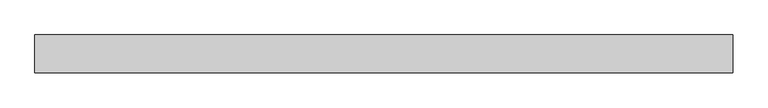
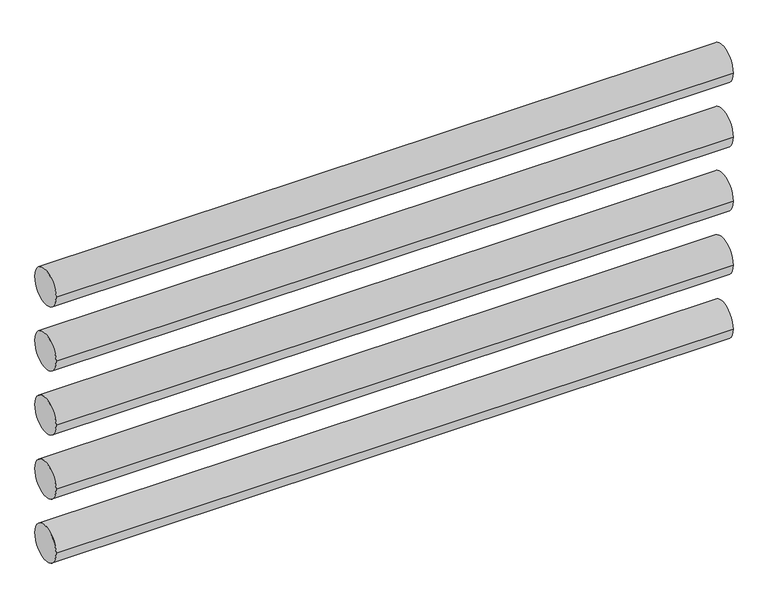
"""IFC4 building model written with IfcOpenShell, lengths in millimetres: proxy geometry, Газпремиум_Регистр : РГТ-2-108х3-2м-5."""

from ifc_helpers import new_model, si_unit, point, frame, frame_2d, origin, place, context, project, spatial, circle_curve, trimmed, segment, composite_curve, outline, extrude, source, transform, mapped, element, save


def mechanical_equipment_43ffbe55(model_context):
    return source(origin(), model_context, "Body", "SweptSolid", [
        extrude(outline(composite_curve([segment(trimmed(circle_curve(frame_2d((0.0, 854.0)), 54.0), [point((-54.0, 854.0))], [point((54.0, 854.0))], False, "CARTESIAN"), True, "CONTINUOUS"), segment(trimmed(circle_curve(frame_2d((0.0, 854.0)), 54.0), [point((54.0, 854.0))], [point((-54.0, 854.0))], False, "CARTESIAN"), True, "CONTINUOUS")], self_intersect=False)), frame((-184.1719207, 0.0, 0.0), z_axis=(1.0, 0.0, 0.0), x_axis=(0.0, 1.0, 0.0)), (0.0, 0.0, 1.0), 2000.0),
        extrude(outline(composite_curve([segment(trimmed(circle_curve(frame_2d((0.0, 654.0)), 54.0), [point((-54.0, 654.0))], [point((54.0, 654.0))], False, "CARTESIAN"), True, "CONTINUOUS"), segment(trimmed(circle_curve(frame_2d((0.0, 654.0)), 54.0), [point((54.0, 654.0))], [point((-54.0, 654.0))], False, "CARTESIAN"), True, "CONTINUOUS")], self_intersect=False)), frame((-184.1719207, 0.0, 0.0), z_axis=(1.0, 0.0, 0.0), x_axis=(0.0, 1.0, 0.0)), (0.0, 0.0, 1.0), 2000.0),
        extrude(outline(composite_curve([segment(trimmed(circle_curve(frame_2d((0.0, 454.0)), 54.0), [point((-54.0, 454.0))], [point((54.0, 454.0))], False, "CARTESIAN"), True, "CONTINUOUS"), segment(trimmed(circle_curve(frame_2d((0.0, 454.0)), 54.0), [point((54.0, 454.0))], [point((-54.0, 454.0))], False, "CARTESIAN"), True, "CONTINUOUS")], self_intersect=False)), frame((-184.1719207, 0.0, 0.0), z_axis=(1.0, 0.0, 0.0), x_axis=(0.0, 1.0, 0.0)), (0.0, 0.0, 1.0), 2000.0),
        extrude(outline(composite_curve([segment(trimmed(circle_curve(frame_2d((0.0, 254.0)), 54.0), [point((-54.0, 254.0))], [point((54.0, 254.0))], False, "CARTESIAN"), True, "CONTINUOUS"), segment(trimmed(circle_curve(frame_2d((0.0, 254.0)), 54.0), [point((54.0, 254.0))], [point((-54.0, 254.0))], False, "CARTESIAN"), True, "CONTINUOUS")], self_intersect=False)), frame((-184.1719207, 0.0, 0.0), z_axis=(1.0, 0.0, 0.0), x_axis=(0.0, 1.0, 0.0)), (0.0, 0.0, 1.0), 2000.0),
        extrude(outline(composite_curve([segment(trimmed(circle_curve(frame_2d((0.0, 54.0)), 54.0), [point((-54.0, 54.0))], [point((54.0, 54.0))], False, "CARTESIAN"), True, "CONTINUOUS"), segment(trimmed(circle_curve(frame_2d((0.0, 54.0)), 54.0), [point((54.0, 54.0))], [point((-54.0, 54.0))], False, "CARTESIAN"), True, "CONTINUOUS")], self_intersect=False)), frame((-184.1719207, 0.0, 0.0), z_axis=(1.0, 0.0, 0.0), x_axis=(0.0, 1.0, 0.0)), (0.0, 0.0, 1.0), 2000.0),
    ])


if __name__ == "__main__":
    model = new_model("IFC4")
    model_context = context("Model", 3, world=origin())
    ifc_project = project(units=[si_unit("LENGTHUNIT", "METRE", prefix="MILLI")], contexts=[model_context])
    site = spatial("IfcSite", under=ifc_project)
    building = spatial("IfcBuilding", under=site)
    placement = place(None, origin())
    mechanical_equipment_shape = mechanical_equipment_43ffbe55(model_context)
    element("IfcBuildingElementProxy", 1, Name="Газпремиум_Регистр : РГТ-2-108х3-2м-5", ObjectType="Газпремиум_Регистр : РГТ-2-108х3-2м-5", at=placement, inside=building, context=model_context, shape_type="MappedRepresentation", body=[
        mapped(mechanical_equipment_shape, transform((0.0, 0.0, 0.0), x_axis=(1.0, 0.0, 0.0), y_axis=(0.0, 1.0, 0.0), z_axis=(0.0, 0.0, 1.0))),
    ])
    save(model, "model.ifc")

# Revit data of these elements
# Type "Газпремиум_Регистр : РГТ-2-108х3-2м-5"
#   ADSK_Позиция = "384"
#   ADSK_Наименование = "Регистр двухрядный из пяти гладких труб 108х3 длиной 2 м, в комплекте с опорами"
#   ADSK_Марка = "РГТ-2-108х3-2м-5-ОП-О ТУ 4936-001-69441315-11"
#   ADSK_Код изделия = "2050884"
#   ADSK_Завод-изготовитель = "ООО ПКП \"ГазПремиум\", Россия, г.Саратов, ИНН 6452951387, кпп 645201001, gaz-premium@mail.ru"
#   ADSK_Единица измерения = "шт."
#   Расстояние между рядами = 200 mm
#   Радиус.регистра = 54 mm
#   Отступ.труб.подкл.от.осевой = 32.719 mm
#   Длина регистра = 2000 mm
#   Диаметр.труб.подкл. = 32 mm
#   Диаметр регистра = 108 mm
#   Высота = 800 mm
#   ADSK_Масса = 181.94
#   ADSK_Количество = 0.5
#   Число рядов = 5
#   Соед.трубы = Грунтовка.красная
#   Регистр = Грунтовка.красная
#   Поддерж.арматура = Грунтовка.серая
#   Default Elevation = 0
# Element 1 (IfcBuildingElementProxy, "Газпремиум_Регистр : РГТ-2-108х3-2м-5")
#   Materials on its faces: "Грунтовка.красная"
# Materials
#   "Грунтовка.красная": class "Разное", colour RGB 255 0 0, transparency 0
#   "Грунтовка.серая": class "Разное", colour RGB 187 181 179, transparency 0
